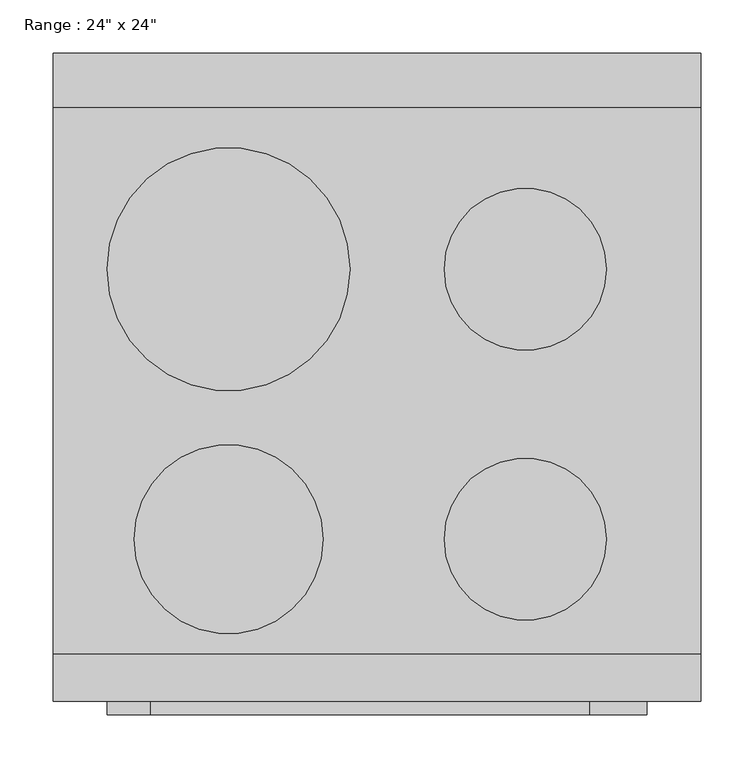
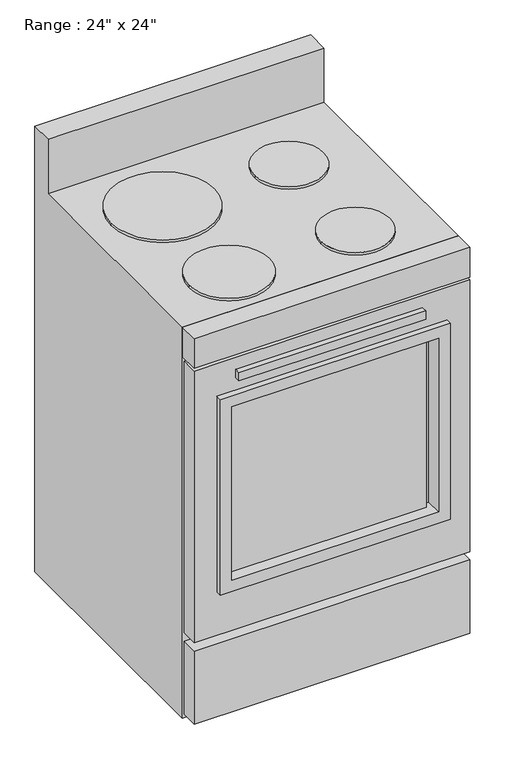
"""IFC4 building model written with IfcOpenShell, lengths in millimetres: proxy geometry."""

from ifc_helpers import new_model, si_unit, point, frame, frame_2d, origin, place, context, project, spatial, polyline, circle_curve, trimmed, segment, composite_curve, outline, extrude, faceted_brep, source, transform, mapped, element, save


def proxy_ce4ccb0f(model_context):
    return source(origin(), model_context, "Body", "SolidModel", [
        faceted_brep([(609.6, 609.6, 0.0), (0.0, 609.6, 0.0), (0.0, 609.6, 1041.4), (609.6, 609.6, 1041.4), (584.2, 609.6, 889.2220355), (25.4, 609.6, 889.2220355), (25.4, 609.6, 254.0), (584.2, 609.6, 254.0), (609.6, 44.45, 914.4), (0.0, 44.45, 914.4), (0.0, 44.45, 0.0), (609.6, 44.45, 0.0), (584.2, 44.45, 889.2220355), (584.2, 44.45, 254.0), (25.4, 44.45, 254.0), (25.4, 44.45, 889.2220355), (609.6, 558.8, 1041.4), (609.6, 558.8, 914.4), (0.0, 558.8, 914.4), (0.0, 558.8, 1041.4)], [[[0, 1, 2, 3], [4, 5, 6, 7]], [[8, 9, 10, 11], [12, 13, 14, 15]], [[0, 3, 16, 17, 8, 11]], [[1, 0, 11, 10]], [[2, 1, 10, 9, 18, 19]], [[9, 8, 17, 18]], [[5, 4, 12, 15]], [[6, 5, 15, 14]], [[7, 6, 14, 13]], [[4, 7, 13, 12]], [[16, 3, 2, 19]], [[17, 16, 19, 18]]]),
        extrude(outline(polyline([(504.825, -12.7), (91.687309, -12.7), (91.687309, 0.0), (504.825, 0.0), (504.825, -12.7)])), frame((0.0, 0.0, 791.2768639), z_axis=(0.0, 0.0, 1.0), x_axis=(1.0, 0.0, 0.0)), (0.0, 0.0, 1.0), 19.05),
        extrude(outline(polyline([(520.7, 12.7), (76.2, 12.7), (76.2, 19.05), (520.7, 19.05), (520.7, 12.7)])), frame((0.0, 0.0, 330.2), z_axis=(0.0, 0.0, 1.0), x_axis=(1.0, 0.0, 0.0)), (0.0, 0.0, 1.0), 406.4),
        extrude(outline(polyline([(609.6, 0.0), (0.0, 0.0), (0.0, 44.45), (609.6, 44.45), (609.6, 0.0)])), frame((0.0, 0.0, 844.7720355), z_axis=(0.0, 0.0, 1.0), x_axis=(1.0, 0.0, 0.0)), (0.0, 0.0, 1.0), 69.6279645),
        extrude(outline(polyline([(762.0, 558.8), (762.0, 50.8), (304.8, 50.8), (304.8, 558.8), (762.0, 558.8)]), holes=[polyline([(736.6, 533.4), (330.2, 533.4), (330.2, 76.2), (736.6, 76.2), (736.6, 533.4)])]), frame((0.0, -12.7, 0.0), z_axis=(0.0, 1.0, 0.0), x_axis=(0.0, 0.0, 1.0)), (0.0, 0.0, 1.0), 38.1),
        extrude(outline(composite_curve([segment(trimmed(circle_curve(frame_2d((165.1, 406.4)), 114.3), [point((50.8, 406.4))], [point((279.4, 406.4))], False, "CARTESIAN"), True, "CONTINUOUS"), segment(trimmed(circle_curve(frame_2d((165.1, 406.4)), 114.3), [point((279.4, 406.4))], [point((50.8, 406.4))], False, "CARTESIAN"), True, "CONTINUOUS")], self_intersect=False)), frame((0.0, 0.0, 914.4), z_axis=(0.0, 0.0, 1.0), x_axis=(1.0, 0.0, 0.0)), (0.0, 0.0, 1.0), 6.35),
        extrude(outline(composite_curve([segment(trimmed(circle_curve(frame_2d((444.5, 406.4)), 76.2), [point((368.3, 406.4))], [point((520.7, 406.4))], False, "CARTESIAN"), True, "CONTINUOUS"), segment(trimmed(circle_curve(frame_2d((444.5, 406.4)), 76.2), [point((520.7, 406.4))], [point((368.3, 406.4))], False, "CARTESIAN"), True, "CONTINUOUS")], self_intersect=False)), frame((0.0, 0.0, 914.4), z_axis=(0.0, 0.0, 1.0), x_axis=(1.0, 0.0, 0.0)), (0.0, 0.0, 1.0), 6.35),
        extrude(outline(composite_curve([segment(trimmed(circle_curve(frame_2d((444.5, 152.4)), 76.2), [point((368.3, 152.4))], [point((520.7, 152.4))], False, "CARTESIAN"), True, "CONTINUOUS"), segment(trimmed(circle_curve(frame_2d((444.5, 152.4)), 76.2), [point((520.7, 152.4))], [point((368.3, 152.4))], False, "CARTESIAN"), True, "CONTINUOUS")], self_intersect=False)), frame((0.0, 0.0, 914.4), z_axis=(0.0, 0.0, 1.0), x_axis=(1.0, 0.0, 0.0)), (0.0, 0.0, 1.0), 6.35),
        extrude(outline(composite_curve([segment(trimmed(circle_curve(frame_2d((165.1, 152.4)), 88.9), [point((76.2, 152.4))], [point((254.0, 152.4))], False, "CARTESIAN"), True, "CONTINUOUS"), segment(trimmed(circle_curve(frame_2d((165.1, 152.4)), 88.9), [point((254.0, 152.4))], [point((76.2, 152.4))], False, "CARTESIAN"), True, "CONTINUOUS")], self_intersect=False)), frame((0.0, 0.0, 914.4), z_axis=(0.0, 0.0, 1.0), x_axis=(1.0, 0.0, 0.0)), (0.0, 0.0, 1.0), 6.35),
        extrude(outline(polyline([(25.4, 609.6), (584.2, 609.6), (584.2, 584.2), (25.4, 584.2), (25.4, 609.6)])), frame((0.0, 0.0, 254.0), z_axis=(0.0, 0.0, 1.0), x_axis=(1.0, 0.0, 0.0)), (0.0, 0.0, 1.0), 635.2220355),
        extrude(outline(polyline([(838.4220355, 609.6), (838.4220355, 0.0), (203.2, 0.0), (203.2, 609.6), (838.4220355, 609.6)]), holes=[polyline([(762.0, 558.8), (304.8, 558.8), (304.8, 50.8), (762.0, 50.8), (762.0, 558.8)])]), frame((0.0, 0.0, 0.0), z_axis=(0.0, 1.0, 0.0), x_axis=(0.0, 0.0, 1.0)), (0.0, 0.0, 1.0), 38.1),
        extrude(outline(polyline([(609.6, 0.0), (0.0, 0.0), (0.0, 38.1), (609.6, 38.1), (609.6, 0.0)])), frame((0.0, 0.0, 12.7), z_axis=(0.0, 0.0, 1.0), x_axis=(1.0, 0.0, 0.0)), (0.0, 0.0, 1.0), 171.45),
    ])


if __name__ == "__main__":
    model = new_model("IFC4")
    model_context = context("Model", 3, world=origin())
    ifc_project = project(units=[si_unit("LENGTHUNIT", "METRE", prefix="MILLI")], contexts=[model_context])
    site = spatial("IfcSite", under=ifc_project)
    building = spatial("IfcBuilding", under=site)
    placement = place(None, origin())
    proxy_shape = proxy_ce4ccb0f(model_context)
    element("IfcBuildingElementProxy", 1, Name="Range : 24\" x 24\"", ObjectType="Range : 24\" x 24\"", at=placement, inside=building, context=model_context, shape_type="MappedRepresentation", body=[
        mapped(proxy_shape, transform((0.0, 0.0, 0.0), x_axis=(1.0, 0.0, 0.0), y_axis=(0.0, 1.0, 0.0), z_axis=(0.0, 0.0, 1.0))),
    ])
    save(model, "model.ifc")

# Revit data of these elements
# Type "Range : 24\" x 24\""
#   Assembly Code = "E1090400"
#   Depth = 2' - 0"
#   Width = 2' - 0"
#   Burner Material = Metal - Chrome
#   Range Material = Metal - Painted Finish - Ivory, Matte
# Element 1 (IfcBuildingElementProxy, "Range : 24\" x 24\"")
#   Materials on its faces: "Metal - Painted Finish - Ivory, Matte", "Metal - Chrome", "TEMPERED INSULATED GLAZING (CARDINAL GLASS LoĒ²-240\nOR EQUIVALENT)"
# Materials
#   "Metal - Chrome": class "Metal", colour RGB 17 17 17, transparency 0
#   "Metal - Painted Finish - Ivory, Matte": class "Paint", colour RGB 247 247 239, transparency 0
#   "TEMPERED INSULATED GLAZING (CARDINAL GLASS LoĒ²-240\nOR EQUIVALENT)": class "Glass", colour RGB 196 205 210, transparency 0.85, Description = "Soda Lime Glass", Cost = 0
